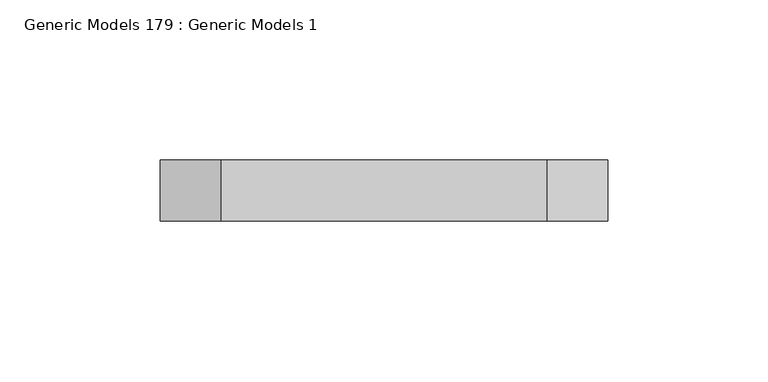
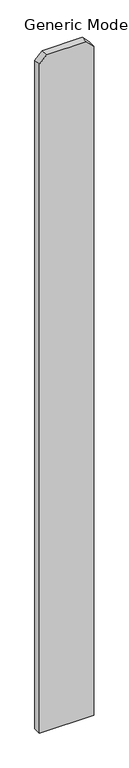
"""IFC4 building model written with IfcOpenShell, lengths in millimetres: proxy geometry, Generic Models 179 : Generic Models 1."""

from ifc_helpers import new_model, si_unit, frame, origin, place, context, project, spatial, polyline, outline, extrude, source, transform, mapped, element, save


def generic_models_179_generic_models_1_ac7d091e(model_context):
    return source(origin(), model_context, "Body", "SweptSolid", [
        extrude(outline(polyline([(76.2, -247829.3875), (1885.95, -247829.3875), (1905.0, -247848.4375), (1905.0, -247950.0375), (1885.95, -247969.0875), (76.2, -247969.0875), (76.2, -247829.3875)])), frame((0.0, 547.6875, 0.0), z_axis=(0.0, 1.0, 0.0), x_axis=(0.0, 0.0, 1.0)), (0.0, 0.0, 1.0), 19.05),
    ])


if __name__ == "__main__":
    model = new_model("IFC4")
    model_context = context("Model", 3, world=origin())
    ifc_project = project(units=[si_unit("LENGTHUNIT", "METRE", prefix="MILLI")], contexts=[model_context])
    site = spatial("IfcSite", under=ifc_project)
    building = spatial("IfcBuilding", under=site)
    placement = place(None, origin())
    generic_models_179_generic_models_1_shape = generic_models_179_generic_models_1_ac7d091e(model_context)
    element("IfcBuildingElementProxy", 1, Name="Generic Models 179 : Generic Models 1", ObjectType="Generic Models 179 : Generic Models 1", at=placement, inside=building, context=model_context, shape_type="MappedRepresentation", body=[
        mapped(generic_models_179_generic_models_1_shape, transform((0.0, 0.0, 0.0), x_axis=(1.0, 0.0, 0.0), y_axis=(0.0, 1.0, 0.0), z_axis=(0.0, 0.0, 1.0))),
    ])
    save(model, "model.ifc")

# Revit data of these elements
# Element 1 (IfcBuildingElementProxy, "Generic Models 179 : Generic Models 1")
#   Materials on its faces: "VERTICAL 1X6 CEDAR PLANKS W/ CLEAR WOOD SEALER"
# Materials
#   "VERTICAL 1X6 CEDAR PLANKS W/ CLEAR WOOD SEALER": class "Wood", colour RGB 234 198 147, transparency 0, Description = "Pinus Echinata", Cost = 0
